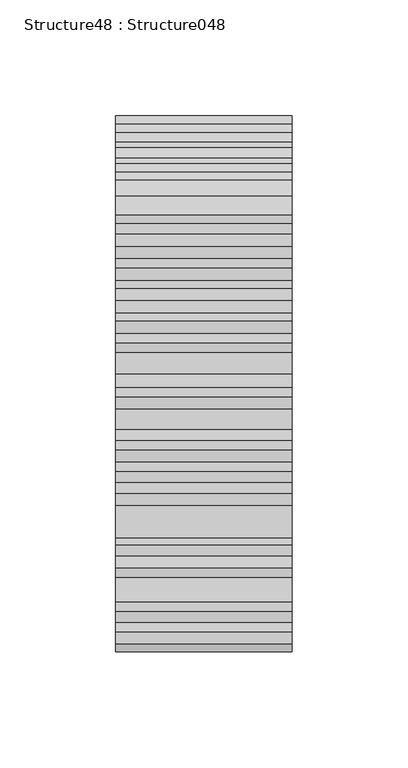
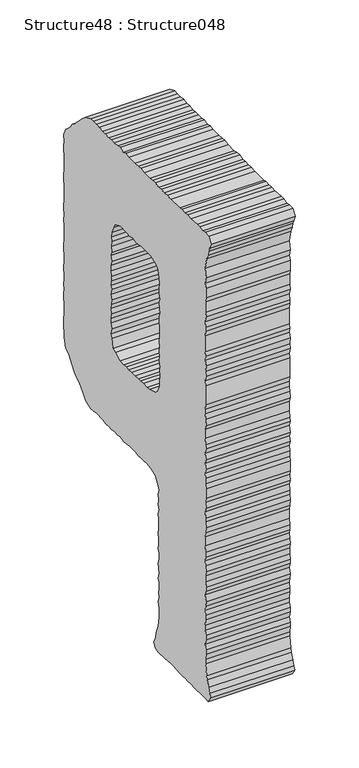
"""IFC4 building model written with IfcOpenShell, lengths in millimetres: proxy geometry, Structure48 : Structure048."""

from ifc_helpers import new_model, si_unit, frame, origin, place, context, project, spatial, polyline, outline, extrude, source, transform, mapped, element, save


def structure48_structure048_e0ce58dd(model_context):
    return source(origin(), model_context, "Body", "SweptSolid", [
        extrude(outline(polyline([(255107.5346057, 3996.390138), (255112.7944992, 3997.5486624), (255116.8942637, 3996.9645864), (255122.7558839, 3996.390138), (255132.1380064, 3996.390138), (255136.2393755, 3997.5486624), (255140.33914, 3996.390138), (255145.621498, 3997.5486624), (255149.1211404, 3996.9645864), (255154.4018938, 3996.9645864), (255159.6842518, 3996.390138), (255163.1838942, 3996.390138), (255168.4646476, 3996.9645864), (255172.5660167, 3996.9645864), (255177.8467701, 3997.5486624), (255183.1066636, 3996.9645864), (255187.7872949, 3996.9645864), (255191.3077972, 3997.5486624), (255199.5089308, 3994.0233463), (255206.5515399, 3987.5792547), (255210.0511823, 3983.4794902), (255213.594149, 3980.5623192), (255215.935267, 3977.6194746), (255220.6142937, 3974.1214368), (255222.9554117, 3970.5768654), (255227.0551762, 3966.5043792), (255230.577283, 3963.5615346), (255234.0753208, 3955.9348494), (255232.9167964, 3950.6765605), (255234.0753208, 3945.4182716), (255234.0753208, 3941.8753048), (255232.9167964, 3936.6186205), (255232.9167964, 3923.1319197), (255234.0753208, 3918.4480792), (255234.0753208, 3912.5896682), (255232.9167964, 3908.46423), (255233.4960586, 3904.3901392), (255232.9167964, 3899.7046941), (255233.4960586, 3893.822214), (255234.0753208, 3889.7208449), (255234.0753208, 3885.0626781), (255233.4960586, 3880.3627915), (255234.0753208, 3874.5043805), (255233.4960586, 3869.8189354), (255232.9167964, 3865.7015202), (255232.9167964, 3856.3161885), (255234.0753208, 3851.6612309), (255234.0753208, 3846.3772683), (255232.9167964, 3841.6741725), (255232.9167964, 3838.1761347), (255234.0753208, 3827.6162325), (255233.4960586, 3822.348316), (255232.9167964, 3818.8310229), (255234.0753208, 3812.9726119), (255233.4960586, 3808.8888934), (255234.0753208, 3804.1890069), (255234.0753208, 3799.5051664), (255233.4960586, 3795.4037973), (255232.9167964, 3790.1294623), (255233.4960586, 3784.8438951), (255234.0753208, 3780.1616592), (255234.0753208, 3771.9605256), (255232.9167964, 3767.2590344), (255232.9167964, 3762.5848215), (255231.1565452, 3753.2171405), (255226.4759139, 3750.8583719), (255224.1364006, 3747.3587295), (255217.0937914, 3739.1592005), (255214.1509468, 3736.2163558), (255209.4719201, 3733.8736333), (255203.6102999, 3726.8566978), (255199.5089308, 3722.1568112), (255191.3077972, 3719.2316172), (255187.7872949, 3719.8140887), (255182.5274014, 3720.4158154), (255172.5660167, 3720.4158154), (255167.8853854, 3719.2316172), (255163.1838942, 3719.8140887), (255158.5032629, 3719.2316172), (255154.981156, 3719.8140887), (255149.1211404, 3719.8140887), (255145.0197713, 3720.4158154), (255139.7598778, 3719.2316172), (255136.2393755, 3719.8140887), (255130.3777553, 3720.4158154), (255121.5973595, 3720.4158154), (255116.3150015, 3719.2316172), (255112.215237, 3719.8140887), (255108.1138679, 3719.8140887), (255103.4332366, 3720.4158154), (255097.5507565, 3719.2316172), (255089.9513496, 3716.8985223), (255087.6102317, 3713.9556777), (255084.0897294, 3706.3289925), (255085.2707183, 3702.229228), (255084.6689916, 3696.3884676), (255085.2707183, 3691.6869765), (255084.0897294, 3687.587212), (255085.2707183, 3683.4858429), (255084.6689916, 3677.6274319), (255084.6689916, 3668.8261762), (255085.2707183, 3664.1423357), (255084.6689916, 3659.4584952), (255084.6689916, 3654.7842823), (255085.2707183, 3649.5003197), (255084.0897294, 3645.9830266), (255084.0897294, 3640.7167147), (255085.2707183, 3636.0408972), (255084.6689916, 3630.7392839), (255084.0897294, 3626.6571701), (255085.2707183, 3621.3732075), (255084.0897294, 3617.8559144), (255084.0897294, 3613.1720739), (255084.6689916, 3607.3393366), (255084.0897294, 3603.7963698), (255085.2707183, 3599.1125293), (255084.0897294, 3593.2541183), (255084.0897294, 3584.4689087), (255085.2707183, 3575.0851816), (255088.1894939, 3569.2524442), (255089.9513496, 3559.8671125), (255092.290863, 3556.3417965), (255089.9513496, 3551.6675836), (255085.2707183, 3550.4833855), (255075.2868691, 3550.4833855), (255070.0269756, 3551.0658569), (255065.9256065, 3551.6675836), (255062.4051042, 3551.6675836), (255051.8644573, 3550.4833855), (255047.7630882, 3550.4833855), (255043.0824569, 3551.0658569), (255038.9826924, 3550.4833855), (255034.2795966, 3551.0658569), (255029.0197031, 3550.4833855), (255024.3182119, 3550.4833855), (255020.8185695, 3551.0658569), (255010.8571848, 3551.0658569), (255006.7558157, 3550.4833855), (255003.2353135, 3556.3417965), (255004.3938379, 3559.8671125), (255006.154089, 3564.54293), (255008.495207, 3570.4109687), (255009.0969337, 3573.9266571), (255010.8571848, 3584.4689087), (255010.8571848, 3588.5702778), (255010.2554581, 3593.8285667), (255010.2554581, 3597.9540049), (255011.436447, 3602.6298224), (255010.2554581, 3607.8961343), (255010.2554581, 3612.0135494), (255011.436447, 3616.0972679), (255011.436447, 3620.7971545), (255010.8571848, 3626.6571701), (255010.8571848, 3630.7392839), (255011.436447, 3635.4407751), (255010.8571848, 3639.5405396), (255010.2554581, 3644.2420307), (255011.436447, 3650.1004418), (255010.2554581, 3654.1841602), (255010.2554581, 3658.3015753), (255010.8571848, 3662.9854159), (255010.8571848, 3668.8261762), (255010.2554581, 3672.9435914), (255010.8571848, 3678.2018803), (255011.436447, 3682.8857208), (255010.8571848, 3686.4030139), (255010.8571848, 3691.0868544), (255011.436447, 3696.9709391), (255011.436447, 3705.7545441), (255010.8571848, 3709.8559132), (255010.2554581, 3715.1302482), (255010.8571848, 3720.4158154), (255010.8571848, 3723.9154578), (255011.436447, 3729.7738688), (255010.2554581, 3733.8736333), (255010.8571848, 3739.1592005), (255010.2554581, 3743.2332913), (255010.2554581, 3752.6170184), (255010.8571848, 3756.7440611), (255010.8571848, 3762.0023501), (255011.436447, 3766.684586), (255010.2554581, 3771.3860772), (255011.436447, 3776.0618947), (255010.2554581, 3780.1616592), (255011.436447, 3786.0280932), (255010.2554581, 3790.7039107), (255010.8571848, 3794.2292268), (255011.436447, 3800.0876378), (255011.436447, 3808.8888934), (255010.2554581, 3812.9726119), (255010.8571848, 3818.8310229), (255011.436447, 3823.5341187), (255011.436447, 3828.2163546), (255010.8571848, 3832.8921721), (255010.8571848, 3851.0595042), (255011.436447, 3855.1769193), (255010.2554581, 3860.4432313), (255010.8571848, 3864.5446004), (255010.2554581, 3870.4030114), (255011.436447, 3875.0772243), (255010.8571848, 3879.1769888), (255011.436447, 3883.2863809), (255011.436447, 3898.5301236), (255010.8571848, 3903.2059411), (255010.8571848, 3906.7328618), (255011.436447, 3912.0071968), (255010.2554581, 3917.2735087), (255010.8571848, 3921.3748778), (255010.8571848, 3931.3346579), (255010.2554581, 3935.4328178), (255010.2554581, 3944.8165449), (255011.436447, 3948.917914), (255010.2554581, 3954.7506513), (255011.436447, 3962.9774586), (255009.0969337, 3973.5197101), (255007.3366826, 3978.2035506), (255006.154089, 3982.8793681), (255004.3938379, 3986.4046842), (255002.6560512, 3991.6806238), (255006.154089, 3996.9645864), (255011.436447, 3997.5486624), (255015.5378161, 3996.390138), (255020.2168428, 3997.5486624), (255024.3182119, 3997.5486624), (255034.8588589, 3996.390138), (255038.9826924, 3997.5486624), (255044.242586, 3996.390138), (255048.9216127, 3996.9645864), (255051.8644573, 3996.390138), (255065.9256065, 3996.390138), (255071.1855, 3996.9645864), (255075.8885958, 3996.390138), (255080.5676225, 3996.9645864), (255084.6689916, 3996.390138), (255089.9513496, 3997.5486624), (255094.0511141, 3997.5486624), (255098.7317454, 3996.390138), (255107.5346057, 3996.390138)]), holes=[polyline([(255089.3720874, 3797.1463977), (255098.7317454, 3794.2292268), (255102.8315099, 3793.6451507), (255108.1138679, 3794.2292268), (255112.7944992, 3793.6451507), (255116.3150015, 3793.6451507), (255121.5973595, 3793.0723069), (255126.857253, 3793.6451507), (255131.5362797, 3793.0723069), (255135.0583866, 3793.6451507), (255139.7598778, 3793.0723069), (255145.0197713, 3793.6451507), (255152.0623804, 3797.1463977), (255156.1637495, 3798.9050443), (255157.9015362, 3807.1045732), (255159.0825251, 3810.6298893), (255157.9015362, 3816.4883003), (255159.0825251, 3821.1737455), (255159.0825251, 3825.849563), (255158.5032629, 3830.5574726), (255159.0825251, 3835.2332901), (255158.5032629, 3839.3587282), (255157.9015362, 3844.0345457), (255159.0825251, 3848.7167816), (255157.9015362, 3854.0007442), (255159.0825251, 3857.5019912), (255158.5032629, 3862.2018778), (255158.5032629, 3866.3032469), (255159.0825251, 3870.9790644), (255159.0825251, 3876.263027), (255157.9015362, 3880.9452629), (255159.0825251, 3886.2051565), (255157.9015362, 3889.7208449), (255158.5032629, 3895.0048075), (255157.9015362, 3900.2887701), (255158.5032629, 3904.3901392), (255157.9015362, 3909.0627475), (255154.981156, 3915.5068392), (255153.2433694, 3919.0321552), (255145.621498, 3921.9733953), (255136.2393755, 3921.9733953), (255130.3777553, 3921.3748778), (255126.2779908, 3922.5494483), (255120.9956328, 3921.3748778), (255117.4959904, 3921.9733953), (255112.7944992, 3922.5494483), (255098.1524832, 3922.5494483), (255089.3720874, 3919.6066036), (255086.4292428, 3916.0909152), (255084.6689916, 3909.0627475), (255084.0897294, 3904.3901392), (255084.6689916, 3899.7046941), (255084.6689916, 3894.4030808), (255083.5104672, 3889.7208449), (255084.6689916, 3886.2051565), (255084.0897294, 3880.3627915), (255083.5104672, 3876.263027), (255084.6689916, 3871.5599312), (255084.6689916, 3867.4601667), (255084.0897294, 3862.8036045), (255084.0897294, 3853.4198774), (255084.6689916, 3848.1166595), (255084.0897294, 3844.6154125), (255084.6689916, 3839.3587282), (255084.0897294, 3834.0474873), (255084.6689916, 3829.9733965), (255083.5104672, 3824.7167122), (255084.0897294, 3821.1737455), (255083.5104672, 3816.4883003), (255084.0897294, 3810.6298893), (255084.0897294, 3805.9476534), (255087.008505, 3799.5051664), (255089.3720874, 3797.1463977)])]), frame((-38594.2176606, 0.0, 0.0), z_axis=(1.0, 0.0, 0.0), x_axis=(0.0, 1.0, 0.0)), (0.0, 0.0, 1.0), 76.2),
    ])


if __name__ == "__main__":
    model = new_model("IFC4")
    model_context = context("Model", 3, world=origin())
    ifc_project = project(units=[si_unit("LENGTHUNIT", "METRE", prefix="MILLI")], contexts=[model_context])
    site = spatial("IfcSite", under=ifc_project)
    building = spatial("IfcBuilding", under=site)
    placement = place(None, origin())
    structure48_structure048_shape = structure48_structure048_e0ce58dd(model_context)
    element("IfcBuildingElementProxy", 1, Name="Structure48 : Structure048", ObjectType="Structure48 : Structure048", at=placement, inside=building, context=model_context, shape_type="MappedRepresentation", body=[
        mapped(structure48_structure048_shape, transform((0.0, 0.0, 0.0), x_axis=(1.0, 0.0, 0.0), y_axis=(0.0, 1.0, 0.0), z_axis=(0.0, 0.0, 1.0))),
    ])
    save(model, "model.ifc")

# Revit data of these elements
# Type "Structure48 : Structure048"
#   NameOverride = "Structure048"
# Element 1 (IfcBuildingElementProxy, "Structure48 : Structure048")
#   Materials on its faces: "BRUSHED ALUM. LETTERING"
# Materials
#   "BRUSHED ALUM. LETTERING": class "Unassigned", colour RGB 169 181 186, transparency 0, Cost = 0
